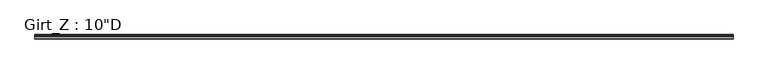
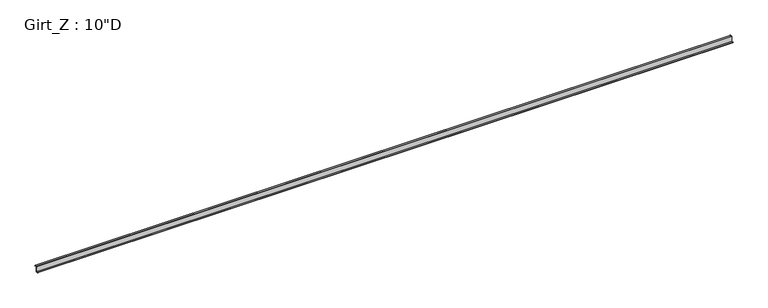
"""IFC4 building model written with IfcOpenShell, lengths in millimetres: beam geometry."""

from ifc_helpers import new_model, si_unit, point, frame, frame_2d, origin, place, context, project, spatial, polyline, circle_curve, trimmed, segment, composite_curve, outline, extrude, source, transform, mapped, element, save


def beam_84a8db34(model_context):
    return source(origin(), model_context, "Body", "SweptSolid", [
        extrude(outline(composite_curve([segment(polyline([(77.9859375, 127.0), (90.2310415, 112.4068534), (88.1028742, 110.621109), (76.6904765, 124.221875), (3.3005807, 124.221875)]), True, "CONTINUOUS"), segment(trimmed(circle_curve(frame_2d((3.3741066, 122.2381931)), 1.9850441), [point((3.3005807, 124.221875))], [point((1.3890625, 122.2381931))], True, "CARTESIAN"), True, "CONTINUOUS"), segment(polyline([(1.3890625, 122.2381931), (1.3890625, -127.0), (-84.3359375, -127.0), (-96.5810415, -112.4068534), (-94.4528742, -110.621109), (-83.0404765, -124.221875), (-3.2694106, -124.221875)]), True, "CONTINUOUS"), segment(trimmed(circle_curve(frame_2d((-3.3748024, -122.2389339)), 1.9857399), [point((-3.2694106, -124.221875))], [point((-1.3890625, -122.2389339))], True, "CARTESIAN"), True, "CONTINUOUS"), segment(polyline([(-1.3890625, -122.2389339), (-1.3890625, 122.2375)]), True, "CONTINUOUS"), segment(trimmed(circle_curve(frame_2d((3.3734375, 122.2375)), 4.7625), [point((-1.3890625, 122.2375))], [point((3.3734375, 127.0))], False, "CARTESIAN"), True, "CONTINUOUS"), segment(polyline([(3.3734375, 127.0), (77.9859375, 127.0)]), True, "CONTINUOUS")], self_intersect=False)), frame((-15635.2875, 0.0, 0.0), z_axis=(1.0, 0.0, 0.0), x_axis=(0.0, 1.0, 0.0)), (0.0, 0.0, 1.0), 31089.6),
    ])


if __name__ == "__main__":
    model = new_model("IFC4")
    model_context = context("Model", 3, world=origin())
    ifc_project = project(units=[si_unit("LENGTHUNIT", "METRE", prefix="MILLI")], contexts=[model_context])
    site = spatial("IfcSite", under=ifc_project)
    building = spatial("IfcBuilding", under=site)
    placement = place(None, origin())
    beam_shape = beam_84a8db34(model_context)
    element("IfcBeam", 1, ObjectType="Girt_Z : 10\"D", at=placement, inside=building, context=model_context, shape_type="MappedRepresentation", body=[
        mapped(beam_shape, transform((0.0, 0.0, 0.0), x_axis=(1.0, 0.0, 0.0), y_axis=(0.0, 1.0, 0.0), z_axis=(0.0, 0.0, 1.0))),
    ])
    save(model, "model.ifc")

# Revit data of these elements
# Type "Girt_Z : 10\"D"
#   half leg = 0' - 1 11/16"
#   Web_Thickness = 0' - 0 7/64"
#   Length [instance default] = 10' - 0"
#   Leg_2 = 0' - 3 3/8"
#   Leg_1 = 0' - 3 1/8"
#   Height = 0' - 10"
#   Structural Material [instance default] = none
# Element 1 (IfcBeam, "Girt_Z : 10\"D")
#   Structural Material = STRUCTURAL STEEL - SEE STRUCT. DWGS
#   Materials on its faces: "STRUCTURAL STEEL - SEE STRUCT. DWGS"
# Materials
#   "STRUCTURAL STEEL - SEE STRUCT. DWGS": class "Metal", colour RGB 137 146 153, transparency 0, Description = "Steel, mill finish", Cost = 0
